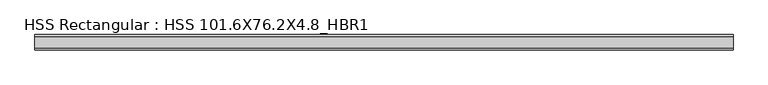
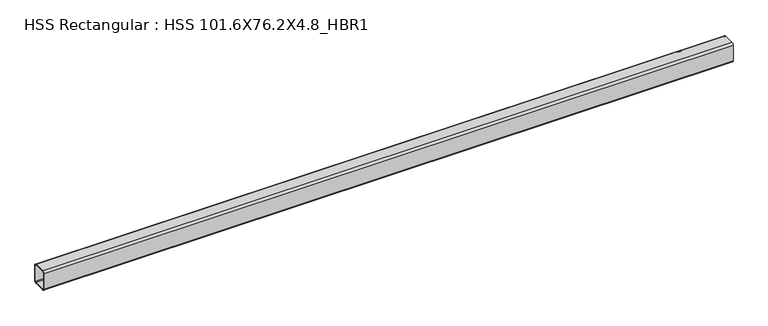
"""IFC4 building model written with IfcOpenShell, lengths in millimetres: beam geometry, HSS Rectangular : HSS 101.6X76.2X4.8_HBR1."""

from ifc_helpers import new_model, si_unit, point, frame, frame_2d, origin, place, context, project, spatial, polyline, circle_curve, trimmed, segment, composite_curve, outline, extrude, source, transform, mapped, element, save


def hss_rectangular_hss_101_6x76_2x4_8_hbr1_eb461c17(model_context):
    return source(origin(), model_context, "Body", "SweptSolid", [
        extrude(outline(composite_curve([segment(polyline([(38.1, 41.275), (38.1, -41.275)]), True, "CONTINUOUS"), segment(trimmed(circle_curve(frame_2d((28.575, -41.275)), 9.525), [point((38.1, -41.275))], [point((28.575, -50.8))], False, "CARTESIAN"), True, "CONTINUOUS"), segment(polyline([(28.575, -50.8), (-28.575, -50.8)]), True, "CONTINUOUS"), segment(trimmed(circle_curve(frame_2d((-28.575, -41.275)), 9.525), [point((-28.575, -50.8))], [point((-38.1, -41.275))], False, "CARTESIAN"), True, "CONTINUOUS"), segment(polyline([(-38.1, -41.275), (-38.1, 41.275)]), True, "CONTINUOUS"), segment(trimmed(circle_curve(frame_2d((-28.575, 41.275)), 9.525), [point((-38.1, 41.275))], [point((-28.575, 50.8))], False, "CARTESIAN"), True, "CONTINUOUS"), segment(polyline([(-28.575, 50.8), (28.575, 50.8)]), True, "CONTINUOUS"), segment(trimmed(circle_curve(frame_2d((28.575, 41.275)), 9.525), [point((28.575, 50.8))], [point((38.1, 41.275))], False, "CARTESIAN"), True, "CONTINUOUS")], self_intersect=False), holes=[composite_curve([segment(trimmed(circle_curve(frame_2d((-28.575, 41.275)), 4.7625), [point((-28.575, 46.0375))], [point((-33.3375, 41.275))], True, "CARTESIAN"), True, "CONTINUOUS"), segment(polyline([(-33.3375, 41.275), (-33.3375, -41.275)]), True, "CONTINUOUS"), segment(trimmed(circle_curve(frame_2d((-28.575, -41.275)), 4.7625), [point((-33.3375, -41.275))], [point((-28.575, -46.0375))], True, "CARTESIAN"), True, "CONTINUOUS"), segment(polyline([(-28.575, -46.0375), (28.575, -46.0375)]), True, "CONTINUOUS"), segment(trimmed(circle_curve(frame_2d((28.575, -41.275)), 4.7625), [point((28.575, -46.0375))], [point((33.3375, -41.275))], True, "CARTESIAN"), True, "CONTINUOUS"), segment(polyline([(33.3375, -41.275), (33.3375, 41.275)]), True, "CONTINUOUS"), segment(trimmed(circle_curve(frame_2d((28.575, 41.275)), 4.7625), [point((33.3375, 41.275))], [point((28.575, 46.0375))], True, "CARTESIAN"), True, "CONTINUOUS"), segment(polyline([(28.575, 46.0375), (-28.575, 46.0375)]), True, "CONTINUOUS")], self_intersect=False)]), frame((-1645.2520459, 0.0, 0.0), z_axis=(1.0, 0.0, 0.0), x_axis=(0.0, 1.0, 0.0)), (0.0, 0.0, 1.0), 3474.9923965),
    ])


if __name__ == "__main__":
    model = new_model("IFC4")
    model_context = context("Model", 3, world=origin())
    ifc_project = project(units=[si_unit("LENGTHUNIT", "METRE", prefix="MILLI")], contexts=[model_context])
    site = spatial("IfcSite", under=ifc_project)
    building = spatial("IfcBuilding", under=site)
    placement = place(None, origin())
    hss_rectangular_hss_101_6x76_2x4_8_hbr1_shape = hss_rectangular_hss_101_6x76_2x4_8_hbr1_eb461c17(model_context)
    element("IfcBeam", 1, ObjectType="HSS Rectangular : HSS 101.6X76.2X4.8_HBR1", at=placement, inside=building, context=model_context, shape_type="MappedRepresentation", body=[
        mapped(hss_rectangular_hss_101_6x76_2x4_8_hbr1_shape, transform((0.0, 0.0, 0.0), x_axis=(1.0, 0.0, 0.0), y_axis=(0.0, 1.0, 0.0), z_axis=(0.0, 0.0, 1.0))),
    ])
    save(model, "model.ifc")

# Revit data of these elements
# Type "HSS Rectangular : HSS 101.6X76.2X4.8_HBR1"
#   Section Name Key = "HSS 4X3X3/16"
#   Assembly Code = "B10"
#   Width = 7.62 cm
#   Wall Nominal Thickness = 0.4763 cm
#   Wall Design Thickness = 0.442 cm
#   Torsional Moment of Inertia = 260.561 cm⁴
#   Torsional Modulus = 61.2876 cm³
#   Section Area = 14.4516 cm²
#   Plastic Modulus weak axis = 40.3122 cm³
#   Plastic Modulus strong axis = 49.1612 cm³
#   Perimeter = 0.881482 m²/m
#   Outer Fillet = 0.9525 cm
#   Nominal Weight = 12.1285 kgf/m
#   Moment of Inertia weak axis = 131.529 cm⁴
#   Moment of Inertia strong axis = 205.202 cm⁴
#   Inner Fillet = 0.4763 cm
#   Height = 10.16 cm
#   Elastic Modulus weak axis = 34.4128 cm³
#   Elastic Modulus strong axis = 40.476 cm³
#   Centroid Vertical = 5.08 cm
#   Centroid Horizontal = 3.81 cm
#   Length [instance default] = 1524 mm
#   Structural Material [instance default] = Steel ASTM A500, Grade B, Rectangular and Square
#   Principal Axes Angle = 0
# Element 1 (IfcBeam, "HSS Rectangular : HSS 101.6X76.2X4.8_HBR1")
#   Structural Material = Steel ASTM A992
#   Materials on its faces: "Steel ASTM A992"
# Materials
#   "Steel ASTM A500, Grade B, Rectangular and Square": class "Metal", colour RGB 199 199 199, transparency 0, Description = "Carbon steel", Cost = 0
#   "Steel ASTM A992": class "Metal", colour RGB 199 199 199, transparency 0, Description = "Structural steel 50ksi", Cost = 0
